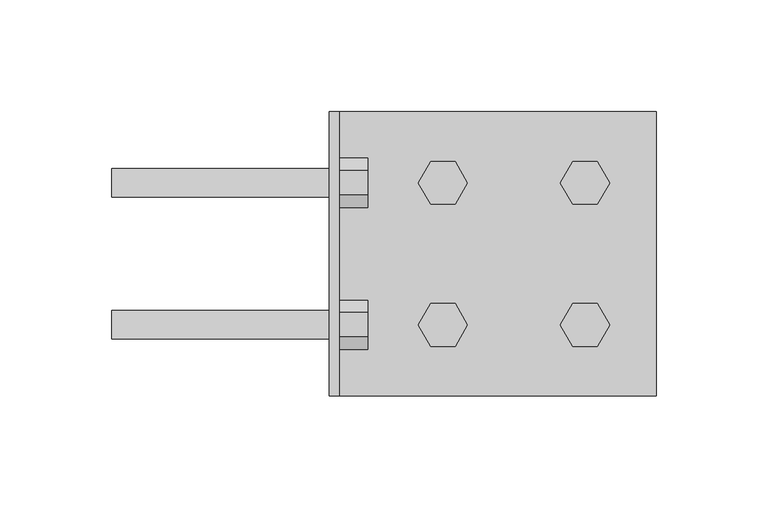
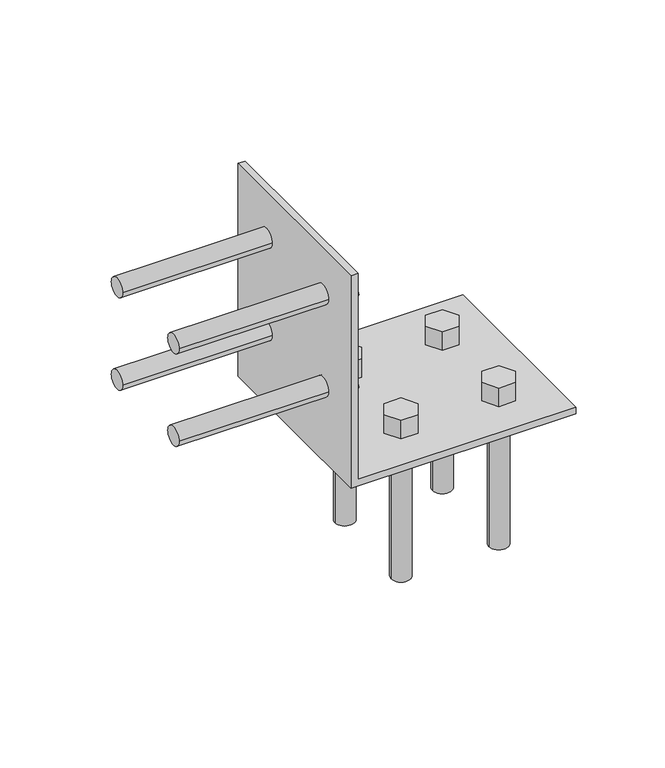
"""IFC4 building model written with IfcOpenShell, lengths in millimetres: fastener geometry."""

from ifc_helpers import new_model, si_unit, point, frame, frame_2d, origin, place, context, project, spatial, polyline, circle_curve, trimmed, segment, composite_curve, outline, extrude, source, transform, mapped, element, save
from ifc_brep_helpers import plane_surface, revolved_surface, advanced_brep


def fastener_979d8faa(model_context):
    return source(origin(), model_context, "Body", "SolidModel", [
        extrude(outline(composite_curve([segment(trimmed(circle_curve(frame_2d((31.75, 50.8)), 6.35), [point((38.1, 50.8))], [point((25.4, 50.8))], False, "CARTESIAN"), True, "CONTINUOUS"), segment(trimmed(circle_curve(frame_2d((31.75, 50.8)), 6.35), [point((25.4, 50.8))], [point((38.1, 50.8))], False, "CARTESIAN"), True, "CONTINUOUS")], self_intersect=False)), frame((-97.0359375, 0.0, 0.0), z_axis=(1.0, 0.0, 0.0), x_axis=(0.0, 1.0, 0.0)), (0.0, 0.0, 1.0), 101.6),
        extrude(outline(polyline([(42.7485226, 50.8), (37.2492613, 41.275), (26.2507387, 41.275), (20.7514774, 50.8), (26.2507387, 60.325), (37.2492613, 60.325), (42.7485226, 50.8)])), frame((4.5640625, 0.0, 0.0), z_axis=(1.0, 0.0, 0.0), x_axis=(0.0, 1.0, 0.0)), (0.0, 0.0, 1.0), 12.7),
        extrude(outline(composite_curve([segment(trimmed(circle_curve(frame_2d((-31.75, 50.8)), 6.35), [point((-25.4, 50.8))], [point((-38.1, 50.8))], False, "CARTESIAN"), True, "CONTINUOUS"), segment(trimmed(circle_curve(frame_2d((-31.75, 50.8)), 6.35), [point((-38.1, 50.8))], [point((-25.4, 50.8))], False, "CARTESIAN"), True, "CONTINUOUS")], self_intersect=False)), frame((-97.0359375, 0.0, 0.0), z_axis=(1.0, 0.0, 0.0), x_axis=(0.0, 1.0, 0.0)), (0.0, 0.0, 1.0), 101.6),
        extrude(outline(polyline([(-20.7514774, 50.8), (-26.2507387, 41.275), (-37.2492613, 41.275), (-42.7485226, 50.8), (-37.2492613, 60.325), (-26.2507387, 60.325), (-20.7514774, 50.8)])), frame((4.5640625, 0.0, 0.0), z_axis=(1.0, 0.0, 0.0), x_axis=(0.0, 1.0, 0.0)), (0.0, 0.0, 1.0), 12.7),
        extrude(outline(composite_curve([segment(trimmed(circle_curve(frame_2d((-31.75, 114.3)), 6.35), [point((-25.4, 114.3))], [point((-38.1, 114.3))], False, "CARTESIAN"), True, "CONTINUOUS"), segment(trimmed(circle_curve(frame_2d((-31.75, 114.3)), 6.35), [point((-38.1, 114.3))], [point((-25.4, 114.3))], False, "CARTESIAN"), True, "CONTINUOUS")], self_intersect=False)), frame((-97.0359375, 0.0, 0.0), z_axis=(1.0, 0.0, 0.0), x_axis=(0.0, 1.0, 0.0)), (0.0, 0.0, 1.0), 101.6),
        extrude(outline(polyline([(-20.7514774, 114.3), (-26.2507387, 104.775), (-37.2492613, 104.775), (-42.7485226, 114.3), (-37.2492613, 123.825), (-26.2507387, 123.825), (-20.7514774, 114.3)])), frame((4.5640625, 0.0, 0.0), z_axis=(1.0, 0.0, 0.0), x_axis=(0.0, 1.0, 0.0)), (0.0, 0.0, 1.0), 12.7),
        extrude(outline(composite_curve([segment(trimmed(circle_curve(frame_2d((31.75, 114.3)), 6.35), [point((38.1, 114.3))], [point((25.4, 114.3))], False, "CARTESIAN"), True, "CONTINUOUS"), segment(trimmed(circle_curve(frame_2d((31.75, 114.3)), 6.35), [point((25.4, 114.3))], [point((38.1, 114.3))], False, "CARTESIAN"), True, "CONTINUOUS")], self_intersect=False)), frame((-97.0359375, 0.0, 0.0), z_axis=(1.0, 0.0, 0.0), x_axis=(0.0, 1.0, 0.0)), (0.0, 0.0, 1.0), 101.6),
        extrude(outline(polyline([(42.7485226, 114.3), (37.2492613, 104.775), (26.2507387, 104.775), (20.7514774, 114.3), (26.2507387, 123.825), (37.2492613, 123.825), (42.7485226, 114.3)])), frame((4.5640625, 0.0, 0.0), z_axis=(1.0, 0.0, 0.0), x_axis=(0.0, 1.0, 0.0)), (0.0, 0.0, 1.0), 12.7),
        extrude(outline(composite_curve([segment(trimmed(circle_curve(frame_2d((50.8, -31.75)), 6.35), [point((44.45, -31.75))], [point((57.15, -31.75))], False, "CARTESIAN"), True, "CONTINUOUS"), segment(trimmed(circle_curve(frame_2d((50.8, -31.75)), 6.35), [point((57.15, -31.75))], [point((44.45, -31.75))], False, "CARTESIAN"), True, "CONTINUOUS")], self_intersect=False)), frame((0.0, 0.0, -97.0359375), z_axis=(0.0, 0.0, 1.0), x_axis=(1.0, 0.0, 0.0)), (0.0, 0.0, 1.0), 101.6),
        extrude(outline(polyline([(39.8014774, -31.75), (45.3007387, -22.225), (56.2992613, -22.225), (61.7985226, -31.75), (56.2992613, -41.275), (45.3007387, -41.275), (39.8014774, -31.75)])), frame((0.0, 0.0, 4.5640625), z_axis=(0.0, 0.0, 1.0), x_axis=(1.0, 0.0, 0.0)), (0.0, 0.0, 1.0), 12.7),
        extrude(outline(composite_curve([segment(trimmed(circle_curve(frame_2d((114.3, -31.75)), 6.35), [point((107.95, -31.75))], [point((120.65, -31.75))], False, "CARTESIAN"), True, "CONTINUOUS"), segment(trimmed(circle_curve(frame_2d((114.3, -31.75)), 6.35), [point((120.65, -31.75))], [point((107.95, -31.75))], False, "CARTESIAN"), True, "CONTINUOUS")], self_intersect=False)), frame((0.0, 0.0, -97.0359375), z_axis=(0.0, 0.0, 1.0), x_axis=(1.0, 0.0, 0.0)), (0.0, 0.0, 1.0), 101.6),
        extrude(outline(polyline([(103.3014774, -31.75), (108.8007387, -22.225), (119.7992613, -22.225), (125.2985226, -31.75), (119.7992613, -41.275), (108.8007387, -41.275), (103.3014774, -31.75)])), frame((0.0, 0.0, 4.5640625), z_axis=(0.0, 0.0, 1.0), x_axis=(1.0, 0.0, 0.0)), (0.0, 0.0, 1.0), 12.7),
        extrude(outline(composite_curve([segment(trimmed(circle_curve(frame_2d((114.3, 31.75)), 6.35), [point((107.95, 31.75))], [point((120.65, 31.75))], False, "CARTESIAN"), True, "CONTINUOUS"), segment(trimmed(circle_curve(frame_2d((114.3, 31.75)), 6.35), [point((120.65, 31.75))], [point((107.95, 31.75))], False, "CARTESIAN"), True, "CONTINUOUS")], self_intersect=False)), frame((0.0, 0.0, -97.0359375), z_axis=(0.0, 0.0, 1.0), x_axis=(1.0, 0.0, 0.0)), (0.0, 0.0, 1.0), 101.6),
        extrude(outline(polyline([(103.3014774, 31.75), (108.8007387, 41.275), (119.7992613, 41.275), (125.2985226, 31.75), (119.7992613, 22.225), (108.8007387, 22.225), (103.3014774, 31.75)])), frame((0.0, 0.0, 4.5640625), z_axis=(0.0, 0.0, 1.0), x_axis=(1.0, 0.0, 0.0)), (0.0, 0.0, 1.0), 12.7),
        extrude(outline(composite_curve([segment(trimmed(circle_curve(frame_2d((50.8, 31.75)), 6.35), [point((44.45, 31.75))], [point((57.15, 31.75))], False, "CARTESIAN"), True, "CONTINUOUS"), segment(trimmed(circle_curve(frame_2d((50.8, 31.75)), 6.35), [point((57.15, 31.75))], [point((44.45, 31.75))], False, "CARTESIAN"), True, "CONTINUOUS")], self_intersect=False)), frame((0.0, 0.0, -97.0359375), z_axis=(0.0, 0.0, 1.0), x_axis=(1.0, 0.0, 0.0)), (0.0, 0.0, 1.0), 101.6),
        extrude(outline(polyline([(39.8014774, 31.75), (45.3007387, 41.275), (56.2992613, 41.275), (61.7985226, 31.75), (56.2992613, 22.225), (45.3007387, 22.225), (39.8014774, 31.75)])), frame((0.0, 0.0, 4.5640625), z_axis=(0.0, 0.0, 1.0), x_axis=(1.0, 0.0, 0.0)), (0.0, 0.0, 1.0), 12.7),
        advanced_brep(
        [(4.5640625, -63.5, 146.05), (4.5640625, -63.5, 4.5640625), (4.5640625, 63.5, 4.5640625), (4.5640625, 63.5, 146.05), (4.5640625, 25.4, 50.8), (4.5640625, 38.1, 50.8), (4.5640625, -38.1, 50.8), (4.5640625, -25.4, 50.8), (4.5640625, -38.1, 114.3), (4.5640625, -25.4, 114.3), (4.5640625, 25.4, 114.3), (4.5640625, 38.1, 114.3), (0.0, 63.5, 146.05), (0.0, 63.5, 0.0), (0.0, -63.5, 0.0), (0.0, -63.5, 146.05), (0.0, 38.1, 50.8), (0.0, 25.4, 50.8), (0.0, -25.4, 50.8), (0.0, -38.1, 50.8), (0.0, -25.4, 114.3), (0.0, -38.1, 114.3), (0.0, 38.1, 114.3), (0.0, 25.4, 114.3), (146.05, 63.5, 4.5640625), (146.05, 63.5, 0.0), (146.05, -63.5, 0.0), (146.05, -63.5, 4.5640625), (57.15, 31.75, 4.5640625), (44.45, 31.75, 4.5640625), (120.65, 31.75, 4.5640625), (107.95, 31.75, 4.5640625), (57.15, -31.75, 4.5640625), (44.45, -31.75, 4.5640625), (120.65, -31.75, 4.5640625), (107.95, -31.75, 4.5640625), (44.45, 31.75, 0.0), (57.15, 31.75, 0.0), (107.95, 31.75, 0.0), (120.65, 31.75, 0.0), (44.45, -31.75, 0.0), (57.15, -31.75, 0.0), (107.95, -31.75, 0.0), (120.65, -31.75, 0.0)],
        [
            (0, 1),
            (1, 2),
            (2, 3),
            (3, 0),
            (4, 5, circle_curve(frame((4.5640625, 31.75, 50.8), z_axis=(-1.0, 0.0, 0.0), x_axis=(0.0, -1.0, 0.0)), 6.35)),
            (5, 4, circle_curve(frame((4.5640625, 31.75, 50.8), z_axis=(-1.0, 0.0, 0.0), x_axis=(0.0, -1.0, 0.0)), 6.35)),
            (6, 7, circle_curve(frame((4.5640625, -31.75, 50.8), z_axis=(-1.0, 0.0, 0.0), x_axis=(0.0, -1.0, 0.0)), 6.35)),
            (7, 6, circle_curve(frame((4.5640625, -31.75, 50.8), z_axis=(-1.0, 0.0, 0.0), x_axis=(0.0, -1.0, 0.0)), 6.35)),
            (8, 9, circle_curve(frame((4.5640625, -31.75, 114.3), z_axis=(-1.0, 0.0, 0.0), x_axis=(0.0, -1.0, 0.0)), 6.35)),
            (9, 8, circle_curve(frame((4.5640625, -31.75, 114.3), z_axis=(-1.0, 0.0, 0.0), x_axis=(0.0, -1.0, 0.0)), 6.35)),
            (10, 11, circle_curve(frame((4.5640625, 31.75, 114.3), z_axis=(-1.0, 0.0, 0.0), x_axis=(0.0, -1.0, 0.0)), 6.35)),
            (11, 10, circle_curve(frame((4.5640625, 31.75, 114.3), z_axis=(-1.0, 0.0, 0.0), x_axis=(0.0, -1.0, 0.0)), 6.35)),
            (12, 13),
            (13, 14),
            (14, 15),
            (15, 12),
            (16, 17, circle_curve(frame((0.0, 31.75, 50.8), z_axis=(1.0, 0.0, 0.0), x_axis=(0.0, -1.0, 0.0)), 6.35)),
            (17, 16, circle_curve(frame((0.0, 31.75, 50.8), z_axis=(1.0, 0.0, 0.0), x_axis=(0.0, -1.0, 0.0)), 6.35)),
            (18, 19, circle_curve(frame((0.0, -31.75, 50.8), z_axis=(1.0, 0.0, 0.0), x_axis=(0.0, -1.0, 0.0)), 6.35)),
            (19, 18, circle_curve(frame((0.0, -31.75, 50.8), z_axis=(1.0, 0.0, 0.0), x_axis=(0.0, -1.0, 0.0)), 6.35)),
            (20, 21, circle_curve(frame((0.0, -31.75, 114.3), z_axis=(1.0, 0.0, 0.0), x_axis=(0.0, -1.0, 0.0)), 6.35)),
            (21, 20, circle_curve(frame((0.0, -31.75, 114.3), z_axis=(1.0, 0.0, 0.0), x_axis=(0.0, -1.0, 0.0)), 6.35)),
            (22, 23, circle_curve(frame((0.0, 31.75, 114.3), z_axis=(1.0, 0.0, 0.0), x_axis=(0.0, -1.0, 0.0)), 6.35)),
            (23, 22, circle_curve(frame((0.0, 31.75, 114.3), z_axis=(1.0, 0.0, 0.0), x_axis=(0.0, -1.0, 0.0)), 6.35)),
            (3, 12),
            (15, 0),
            (2, 24),
            (24, 25),
            (25, 13),
            (14, 26),
            (26, 27),
            (27, 1),
            (27, 24),
            (28, 29, circle_curve(frame((50.8, 31.75, 4.5640625), z_axis=(0.0, 0.0, -1.0), x_axis=(1.0, 0.0, 0.0)), 6.35)),
            (29, 28, circle_curve(frame((50.8, 31.75, 4.5640625), z_axis=(0.0, 0.0, -1.0), x_axis=(1.0, 0.0, 0.0)), 6.35)),
            (30, 31, circle_curve(frame((114.3, 31.75, 4.5640625), z_axis=(0.0, 0.0, -1.0), x_axis=(1.0, 0.0, 0.0)), 6.35)),
            (31, 30, circle_curve(frame((114.3, 31.75, 4.5640625), z_axis=(0.0, 0.0, -1.0), x_axis=(1.0, 0.0, 0.0)), 6.35)),
            (32, 33, circle_curve(frame((50.8, -31.75, 4.5640625), z_axis=(0.0, 0.0, -1.0), x_axis=(1.0, 0.0, 0.0)), 6.35)),
            (33, 32, circle_curve(frame((50.8, -31.75, 4.5640625), z_axis=(0.0, 0.0, -1.0), x_axis=(1.0, 0.0, 0.0)), 6.35)),
            (34, 35, circle_curve(frame((114.3, -31.75, 4.5640625), z_axis=(0.0, 0.0, -1.0), x_axis=(1.0, 0.0, 0.0)), 6.35)),
            (35, 34, circle_curve(frame((114.3, -31.75, 4.5640625), z_axis=(0.0, 0.0, -1.0), x_axis=(1.0, 0.0, 0.0)), 6.35)),
            (25, 26),
            (36, 37, circle_curve(frame((50.8, 31.75, 0.0), z_axis=(0.0, 0.0, 1.0), x_axis=(1.0, 0.0, 0.0)), 6.35)),
            (37, 36, circle_curve(frame((50.8, 31.75, 0.0), z_axis=(0.0, 0.0, 1.0), x_axis=(1.0, 0.0, 0.0)), 6.35)),
            (38, 39, circle_curve(frame((114.3, 31.75, 0.0), z_axis=(0.0, 0.0, 1.0), x_axis=(1.0, 0.0, 0.0)), 6.35)),
            (39, 38, circle_curve(frame((114.3, 31.75, 0.0), z_axis=(0.0, 0.0, 1.0), x_axis=(1.0, 0.0, 0.0)), 6.35)),
            (40, 41, circle_curve(frame((50.8, -31.75, 0.0), z_axis=(0.0, 0.0, 1.0), x_axis=(1.0, 0.0, 0.0)), 6.35)),
            (41, 40, circle_curve(frame((50.8, -31.75, 0.0), z_axis=(0.0, 0.0, 1.0), x_axis=(1.0, 0.0, 0.0)), 6.35)),
            (42, 43, circle_curve(frame((114.3, -31.75, 0.0), z_axis=(0.0, 0.0, 1.0), x_axis=(1.0, 0.0, 0.0)), 6.35)),
            (43, 42, circle_curve(frame((114.3, -31.75, 0.0), z_axis=(0.0, 0.0, 1.0), x_axis=(1.0, 0.0, 0.0)), 6.35)),
            (29, 36),
            (37, 28),
            (39, 30),
            (31, 38),
            (41, 32),
            (33, 40),
            (43, 34),
            (35, 42),
            (5, 16),
            (17, 4),
            (19, 6),
            (7, 18),
            (21, 8),
            (9, 20),
            (23, 10),
            (11, 22),
        ],
        [
            plane_surface(frame((4.5640625, 63.5, 146.05), z_axis=(1.0, 0.0, 0.0), x_axis=(0.0, 1.0, 0.0))),
            plane_surface(frame((0.0, 63.5, 146.05), z_axis=(-1.0, 0.0, 0.0), x_axis=(0.0, -1.0, 0.0))),
            plane_surface(frame((4.5640625, -63.5, 146.05), z_axis=(0.0, 0.0, 1.0), x_axis=(-1.0, 0.0, 0.0))),
            plane_surface(frame((4.5640625, 63.5, 146.05), z_axis=(0.0, 1.0, 0.0), x_axis=(-1.0, 0.0, 0.0))),
            plane_surface(frame((4.5640625, -63.5, 4.5640625), z_axis=(0.0, -1.0, 0.0), x_axis=(-1.0, 0.0, 0.0))),
            plane_surface(frame((0.0, -63.5, 4.5640625), z_axis=(0.0, 0.0, 1.0), x_axis=(-1.0, 0.0, 0.0))),
            plane_surface(frame((0.0, -63.5, 0.0), z_axis=(0.0, 0.0, -1.0), x_axis=(1.0, 0.0, 0.0))),
            plane_surface(frame((146.05, 63.5, 4.5640625), z_axis=(1.0, 0.0, 0.0), x_axis=(0.0, 0.0, -1.0))),
            revolved_surface(polyline([(57.15, 31.75, 4.5640625), (57.15, 31.75, 0.0)]), (50.8, 31.75, 0.0), (0.0, 0.0, 1.0)),
            revolved_surface(polyline([(120.64999999999999, 31.75, 4.5640625), (120.64999999999999, 31.75, 0.0)]), (114.3, 31.75, 0.0), (0.0, 0.0, 1.0)),
            revolved_surface(polyline([(57.15, -31.75, 4.5640625), (57.15, -31.75, 0.0)]), (50.8, -31.75, 0.0), (0.0, 0.0, 1.0)),
            revolved_surface(polyline([(120.64999999999999, -31.75, 4.5640625), (120.64999999999999, -31.75, 0.0)]), (114.3, -31.75, 0.0), (0.0, 0.0, 1.0)),
            revolved_surface(polyline([(4.5640625, 25.4, 50.8), (0.0, 25.4, 50.8)]), (0.0, 31.75, 50.8), (1.0, 0.0, 0.0)),
            revolved_surface(polyline([(4.5640625, -38.1, 50.8), (0.0, -38.1, 50.8)]), (0.0, -31.75, 50.8), (1.0, 0.0, 0.0)),
            revolved_surface(polyline([(4.5640625, -38.1, 114.3), (0.0, -38.1, 114.3)]), (0.0, -31.75, 114.3), (1.0, 0.0, 0.0)),
            revolved_surface(polyline([(4.5640625, 25.4, 114.3), (0.0, 25.4, 114.3)]), (0.0, 31.75, 114.3), (1.0, 0.0, 0.0)),
        ],
        [
            (0, [[1, 2, 3, 4], [5, 6], [7, 8], [9, 10], [11, 12]]),
            (1, [[13, 14, 15, 16], [17, 18], [19, 20], [21, 22], [23, 24]]),
            (2, [[25, -16, 26, -4]]),
            (3, [[27, 28, 29, -13, -25, -3]]),
            (4, [[-26, -15, 30, 31, 32, -1]]),
            (5, [[-27, -2, -32, 33], [34, 35], [36, 37], [38, 39], [40, 41]]),
            (6, [[-30, -14, -29, 42], [43, 44], [45, 46], [47, 48], [49, 50]]),
            (7, [[-31, -42, -28, -33]]),
            (8, [[-35, 51, -44, 52]]),
            (8, [[-43, -51, -34, -52]]),
            (9, [[-46, 53, -37, 54]]),
            (9, [[-36, -53, -45, -54]]),
            (10, [[-48, 55, -39, 56]]),
            (10, [[-38, -55, -47, -56]]),
            (11, [[-50, 57, -41, 58]]),
            (11, [[-40, -57, -49, -58]]),
            (12, [[-6, 59, -18, 60]]),
            (12, [[-17, -59, -5, -60]]),
            (13, [[-20, 61, -8, 62]]),
            (13, [[-7, -61, -19, -62]]),
            (14, [[-22, 63, -10, 64]]),
            (14, [[-9, -63, -21, -64]]),
            (15, [[-24, 65, -12, 66]]),
            (15, [[-11, -65, -23, -66]]),
        ],
    ),
    ])


if __name__ == "__main__":
    model = new_model("IFC4")
    model_context = context("Model", 3, world=origin())
    ifc_project = project(units=[si_unit("LENGTHUNIT", "METRE", prefix="MILLI")], contexts=[model_context])
    site = spatial("IfcSite", under=ifc_project)
    building = spatial("IfcBuilding", under=site)
    placement = place(None, origin())
    fastener_shape = fastener_979d8faa(model_context)
    element("IfcFastener", 1, ObjectType="SIMPSON - HLPC/HLGPC Heavy Angles and Gussets : SIMPSON -HL55 - 5 X 5.75 - .5\" BOLT - HDG", at=placement, inside=building, context=model_context, shape_type="MappedRepresentation", body=[
        mapped(fastener_shape, transform((0.0, 0.0, 0.0), x_axis=(1.0, 0.0, 0.0), y_axis=(0.0, 1.0, 0.0), z_axis=(0.0, 0.0, 1.0))),
    ])
    save(model, "model.ifc")

# Revit data of these elements
# Type "SIMPSON - HLPC/HLGPC Heavy Angles and Gussets : SIMPSON -HL55 - 5 X 5.75 - .5\" BOLT - HDG"
#   URL = "https://www.strongtie.com/classiccollection_architecturalproductsgroup/hlpc-hlgpc_productgroup_wcc/p/hlpc.hlgpc"
#   L = 0' - 5"
#   Hole Radius = 0' - 0 1/4"
#   D4 = 0' - 2 1/2"
#   D2 = 0' - 2 1/2"
#   D1 = 0' - 1 1/4"
#   D3 = 0' - 2"
#   Ga. = 0' - 0 23/128"
#   W1 & W2 = 0' - 5 3/4"
#   Default Elevation = 4' - 0"
#   Bolt Visibility - 3B = no
#   Bolt Visibility - 3A = no
#   Bolt Visibility - 2B = yes
#   Bolt Visibility - 2A = yes
#   Bolt Visibility - 1B = yes
#   Bolt Visibility - 1A = yes
#   Bolt Visibility = yes
#   Bolt Size = element 1298416
# Element 1 (IfcFastener, "SIMPSON - HLPC/HLGPC Heavy Angles and Gussets : SIMPSON -HL55 - 5 X 5.75 - .5\" BOLT - HDG")
#   Materials on its faces: "1/2\" X 5\" LAG BOLT (THRU BOLT IF PLATE ON OPP. SIDE OF STRUCT MEMBER)"
# Materials
#   "1/2\" X 5\" LAG BOLT (THRU BOLT IF PLATE ON OPP. SIDE OF STRUCT MEMBER)": class "Generic", colour RGB 120 120 120, transparency 0, Cost = 0
